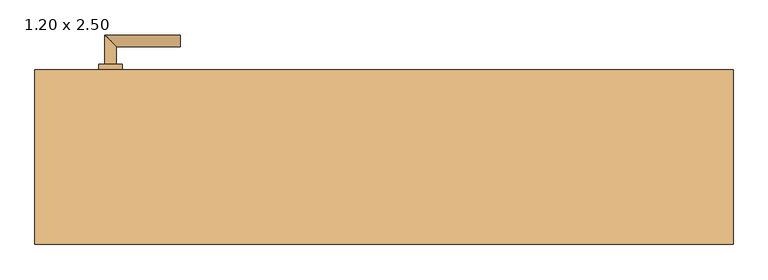
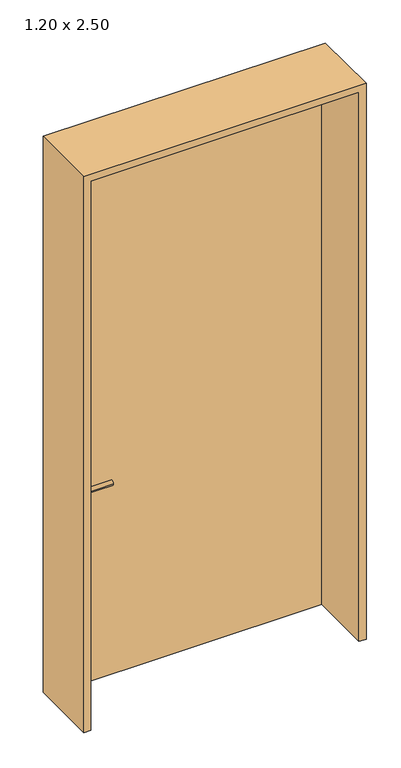
"""IFC4 building model written with IfcOpenShell, lengths in millimetres: door geometry, Drehflügel 1-flg - Blockzarge : 1.20 x 2.50."""

from ifc_helpers import new_model, si_unit, point, frame, frame_2d, origin, place, context, project, spatial, polyline, circle_curve, ellipse_curve, trimmed, segment, composite_curve, outline, extrude, source, transform, mapped, element, save
from ifc_brep_helpers import plane_surface, cylinder_surface, advanced_brep


def door_1_20_x_2_50_48e01e02(model_context):
    return source(origin(), model_context, "Body", "SolidModel", [
        advanced_brep(
        [(-460.0, 129.4346141, 1000.0), (-480.0, 129.4346141, 1000.0), (-460.0, 99.4346141, 1000.0), (-480.0, 79.4346141, 1000.0), (-350.0, 99.4346141, 1000.0), (-350.0, 79.4346141, 1000.0)],
        [
            (0, 1, circle_curve(frame((-470.0, 129.4346141, 1000.0), z_axis=(0.0, 1.0, 0.0), x_axis=(-1.0, 0.0, 0.0)), 10.0)),
            (1, 0, circle_curve(frame((-470.0, 129.4346141, 1000.0), z_axis=(0.0, 1.0, 0.0), x_axis=(-1.0, 0.0, 0.0)), 10.0)),
            (0, 2),
            (2, 3, ellipse_curve(frame((-470.0, 89.4346141, 1000.0), z_axis=(-0.7071067811865686, 0.7071067811865265, 0.0), x_axis=(0.7071067811865264, 0.7071067811865687, 0.0)), 14.1421356, 10.0)),
            (3, 1),
            (3, 2, ellipse_curve(frame((-470.0, 89.4346141, 1000.0), z_axis=(-0.7071067811865686, 0.7071067811865265, 0.0), x_axis=(0.7071067811865264, 0.7071067811865687, 0.0)), 14.1421356, 10.0)),
            (4, 5, circle_curve(frame((-350.0, 89.4346141, 1000.0), z_axis=(1.0, 0.0, 0.0), x_axis=(0.0, -1.0, 0.0)), 10.0)),
            (5, 4, circle_curve(frame((-350.0, 89.4346141, 1000.0), z_axis=(1.0, 0.0, 0.0), x_axis=(0.0, -1.0, 0.0)), 10.0)),
            (2, 4),
            (5, 3),
        ],
        [
            plane_surface(frame((-470.0, 129.4346141, -287.7526403), z_axis=(0.0, 1.0, 0.0), x_axis=(0.0, 0.0, 1.0))),
            cylinder_surface(frame((-470.0, 129.4346141, 1000.0), z_axis=(0.0, 1.0, 0.0), x_axis=(-1.0, 0.0, 0.0)), 10.0),
            plane_surface(frame((-350.0, 89.4346141, -287.7526403), z_axis=(1.0, 0.0, 0.0), x_axis=(0.0, 0.0, 1.0))),
            cylinder_surface(frame((-470.0, 89.4346141, 1000.0), z_axis=(-1.0, 0.0, 0.0), x_axis=(0.0, -1.0, 0.0)), 10.0),
        ],
        [
            (0, [[1, 2]]),
            (1, [[-1, 3, 4, 5]]),
            (1, [[-2, -5, 6, -3]]),
            (2, [[7, 8]]),
            (3, [[-4, 9, -8, 10]]),
            (3, [[-6, -10, -7, -9]]),
        ],
    ),
        advanced_brep(
        [(-460.0, 174.4346141, 1000.0), (-480.0, 174.4346141, 1000.0), (-460.0, 204.4346141, 1000.0), (-480.0, 224.4346141, 1000.0), (-350.0, 204.4346141, 1000.0), (-350.0, 224.4346141, 1000.0)],
        [
            (0, 1, circle_curve(frame((-470.0, 174.4346141, 1000.0), z_axis=(0.0, -1.0, 0.0), x_axis=(-1.0, 0.0, 0.0)), 10.0)),
            (1, 0, circle_curve(frame((-470.0, 174.4346141, 1000.0), z_axis=(0.0, -1.0, 0.0), x_axis=(-1.0, 0.0, 0.0)), 10.0)),
            (0, 2),
            (2, 3, ellipse_curve(frame((-470.0, 214.4346141, 1000.0), z_axis=(-0.7071067811865486, -0.7071067811865464, 0.0), x_axis=(0.7071067811865464, -0.7071067811865488, 0.0)), 14.1421356, 10.0)),
            (3, 1),
            (3, 2, ellipse_curve(frame((-470.0, 214.4346141, 1000.0), z_axis=(-0.7071067811865486, -0.7071067811865464, 0.0), x_axis=(0.7071067811865464, -0.7071067811865488, 0.0)), 14.1421356, 10.0)),
            (4, 5, circle_curve(frame((-350.0, 214.4346141, 1000.0), z_axis=(1.0, 0.0, 0.0), x_axis=(0.0, 1.0, 0.0)), 10.0)),
            (5, 4, circle_curve(frame((-350.0, 214.4346141, 1000.0), z_axis=(1.0, 0.0, 0.0), x_axis=(0.0, 1.0, 0.0)), 10.0)),
            (2, 4),
            (5, 3),
        ],
        [
            plane_surface(frame((-470.0, 174.4346141, -287.7526403), z_axis=(0.0, -1.0, 0.0), x_axis=(0.0, 0.0, 1.0))),
            cylinder_surface(frame((-470.0, 174.4346141, 1000.0), z_axis=(0.0, -1.0, 0.0), x_axis=(-1.0, 0.0, 0.0)), 10.0),
            plane_surface(frame((-350.0, 214.4346141, -287.7526403), z_axis=(1.0, 0.0, 0.0), x_axis=(0.0, 0.0, 1.0))),
            cylinder_surface(frame((-470.0, 214.4346141, 1000.0), z_axis=(-1.0, 0.0, 0.0), x_axis=(0.0, 1.0, 0.0)), 10.0),
        ],
        [
            (0, [[1, 2]]),
            (1, [[-1, 3, 4, 5]]),
            (1, [[-2, -5, 6, -3]]),
            (2, [[7, 8]]),
            (3, [[-4, 9, -8, 10]]),
            (3, [[-6, -10, -7, -9]]),
        ],
    ),
        extrude(outline(composite_curve([segment(trimmed(circle_curve(frame_2d((1000.0, -470.0)), 20.0), [point((1000.0, -450.0))], [point((1000.0, -490.0))], False, "CARTESIAN"), True, "CONTINUOUS"), segment(trimmed(circle_curve(frame_2d((1000.0, -470.0)), 20.0), [point((1000.0, -490.0))], [point((1000.0, -450.0))], False, "CARTESIAN"), True, "CONTINUOUS")], self_intersect=False)), frame((0.0, 129.4346141, 0.0), z_axis=(0.0, 1.0, 0.0), x_axis=(0.0, 0.0, 1.0)), (0.0, 0.0, 1.0), 10.0),
        extrude(outline(composite_curve([segment(trimmed(circle_curve(frame_2d((1000.0, -470.0)), 20.0), [point((1000.0, -450.0))], [point((1000.0, -490.0))], False, "CARTESIAN"), True, "CONTINUOUS"), segment(trimmed(circle_curve(frame_2d((1000.0, -470.0)), 20.0), [point((1000.0, -490.0))], [point((1000.0, -450.0))], False, "CARTESIAN"), True, "CONTINUOUS")], self_intersect=False)), frame((0.0, 164.4346141, 0.0), z_axis=(0.0, 1.0, 0.0), x_axis=(0.0, 0.0, 1.0)), (0.0, 0.0, 1.0), 10.0),
        extrude(outline(polyline([(2600.0, 600.0), (2600.0, -600.0), (100.0, -600.0), (100.0, -570.0), (2570.0, -570.0), (2570.0, 570.0), (100.0, 570.0), (100.0, 600.0), (2600.0, 600.0)])), frame((0.0, -135.5653859, 0.0), z_axis=(0.0, 1.0, 0.0), x_axis=(0.0, 0.0, 1.0)), (0.0, 0.0, 1.0), 300.0),
        extrude(outline(polyline([(570.0, 164.4346141), (570.0, 139.4346141), (-570.0, 139.4346141), (-570.0, 164.4346141), (570.0, 164.4346141)])), frame((0.0, 0.0, 100.0), z_axis=(0.0, 0.0, 1.0), x_axis=(1.0, 0.0, 0.0)), (0.0, 0.0, 1.0), 2470.0),
    ])


if __name__ == "__main__":
    model = new_model("IFC4")
    model_context = context("Model", 3, world=origin())
    ifc_project = project(units=[si_unit("LENGTHUNIT", "METRE", prefix="MILLI")], contexts=[model_context])
    site = spatial("IfcSite", under=ifc_project)
    building = spatial("IfcBuilding", under=site)
    placement = place(None, origin())
    door_1_20_x_2_50_shape = door_1_20_x_2_50_48e01e02(model_context)
    element("IfcDoor", 1, ObjectType="Drehflügel 1-flg - Blockzarge : 1.20 x 2.50", at=placement, inside=building, context=model_context, shape_type="MappedRepresentation", body=[
        mapped(door_1_20_x_2_50_shape, transform((0.0, 0.0, 0.0), x_axis=(1.0, 0.0, 0.0), y_axis=(0.0, 1.0, 0.0), z_axis=(0.0, 0.0, 1.0))),
    ])
    save(model, "model.ifc")

# Revit data of these elements
# Type "Drehflügel 1-flg - Blockzarge : 1.20 x 2.50"
#   Type Mark = "27"
#   Operation = "SingleSwingRight"
#   Keynote = "16.03"
#   Visual Light Transmittance = 0.9
#   Solar Heat Gain Coefficient = 0.86
#   Heat Transfer Coefficient (U) = 5.5617 W/(m²·K)
#   Rough Width = 1.200 m
#   Stärke Futter = 0.030 m
#   Rough Height [instance default] = 2.600 m
#   Höhe Türgriff = 0.900 m
#   Height = 2.500 m
#   Fußbodenaufbau [instance default] = 0.100 m
#   Width = 1.200 m
#   Sichtbarkeit Sturzlinien [instance default] = yes
#   Türgriff auswählen [instance default] = element 420047
#   Türgriff [instance default] = none
#   Türflügel [instance default] = none
#   Rahmen/Pfosten [instance default] = none
#   Construction Type Id = ""
#   Function = (empty or 0)
#   Wall Closure = (empty or 0)
#   Analytic Construction = (empty or 0)
# Element 1 (IfcDoor, "Drehflügel 1-flg - Blockzarge : 1.20 x 2.50")
#   Materials on its faces: "Metall - Chrom", "Holz - Birke"
# Materials
#   "Metall - Chrom": class "Metall", colour RGB 247 247 247, transparency 0, Cost = 0
#   "Holz - Birke": class "Holz", colour RGB 213 164 103, transparency 0, Cost = 0
